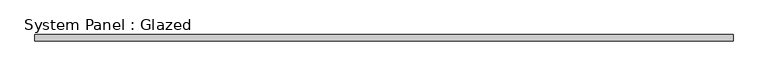
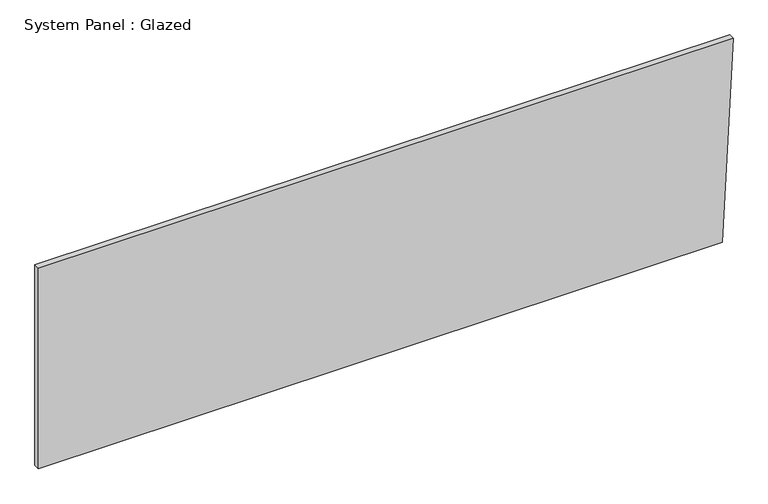
"""IFC4 building model written with IfcOpenShell, lengths in millimetres: plate geometry, System Panel : Glazed."""

import ifcopenshell
import ifcopenshell.guid

model = None  # the IFC model being written
_history = None  # IfcOwnerHistory: only IFC2X3 demands one
_inside = {}  # id of a spatial element -> (the spatial element, [elements in it])
_under = {}  # id of a project, library or spatial element -> (it, [spatial elements below it])
_declared = {}  # id of a project -> (the project, [libraries it declares])
_typed = {}  # id of a type object -> (the type object, [elements of that type])
_made_of = {}  # id of a material, layer set ... -> (it, [elements and type objects made of it])


def new_model(schema):
    """Start an empty IFC model of exactly this schema.

    Asked for "IFC4X3", IfcOpenShell would pick the latest addendum, in which some entities
    have other attributes; the version numbers below select the first issue.
    IFC2X3 requires an IfcOwnerHistory on every rooted entity: one is made here for all.
    """
    global model, _history
    if schema == "IFC4X3":
        model = ifcopenshell.file(schema_version=(4, 3, 0, 0))
    else:
        model = ifcopenshell.file(schema=schema)
    _inside.clear()
    _under.clear()
    _declared.clear()
    _typed.clear()
    _made_of.clear()
    _history = None
    if model.schema == "IFC2X3":
        org = make("IfcOrganization", Name="unknown")
        user = make(
            "IfcPersonAndOrganization",
            ThePerson=make("IfcPerson", FamilyName="unknown"),
            TheOrganization=org,
        )
        app = make(
            "IfcApplication",
            ApplicationDeveloper=org,
            Version="unknown",
            ApplicationFullName="unknown",
            ApplicationIdentifier="unknown",
        )
        _history = make(
            "IfcOwnerHistory",
            OwningUser=user,
            OwningApplication=app,
            ChangeAction="ADDED",
            CreationDate=0,
        )
    return model


def make(cls, **values):
    """One entity of the class cls with the attributes given. An attribute that is None is left unset."""
    return model.create_entity(
        cls, **{name: value for name, value in values.items() if value is not None}
    )


def rooted(cls, **values):
    """An entity with a GlobalId (a new one), such as an element, a storey or a relation."""
    return make(cls, GlobalId=ifcopenshell.guid.new(), OwnerHistory=_history, **values)


def si_unit(unit_type, name, prefix=None):
    """IfcSIUnit, for example si_unit("LENGTHUNIT", "METRE", prefix="MILLI")."""
    return make("IfcSIUnit", UnitType=unit_type, Prefix=prefix, Name=name)


def assignment(units):
    """IfcUnitAssignment: the units of a project."""
    return None if units is None else make("IfcUnitAssignment", Units=units)


def point(xyz):
    """IfcCartesianPoint."""
    return None if xyz is None else make("IfcCartesianPoint", Coordinates=xyz)


def direction(xyz):
    """IfcDirection."""
    return None if xyz is None else make("IfcDirection", DirectionRatios=xyz)


def frame(location, z_axis=None, x_axis=None):
    """IfcAxis2Placement3D, a coordinate frame: its origin and axes. An axis left out is left unset."""
    return make(
        "IfcAxis2Placement3D",
        Location=point(location),
        Axis=direction(z_axis),
        RefDirection=direction(x_axis),
    )


def origin():
    """The frame at (0, 0, 0) with its axes left unset."""
    return frame((0.0, 0.0, 0.0))


def place(relative_to, where):
    """IfcLocalPlacement: puts the frame where relative to a parent placement (None: the world)."""
    return make(
        "IfcLocalPlacement", PlacementRelTo=relative_to, RelativePlacement=where
    )


def context(
    kind, dimensions, precision=None, world=None, true_north=None, identifier=None
):
    """IfcGeometricRepresentationContext, for example the 3D "Model" context."""
    return make(
        "IfcGeometricRepresentationContext",
        ContextIdentifier=identifier,
        ContextType=kind,
        CoordinateSpaceDimension=dimensions,
        Precision=precision,
        WorldCoordinateSystem=world,
        TrueNorth=true_north,
    )


def project(units=None, contexts=None):
    """IfcProject with its units and contexts."""
    return rooted(
        "IfcProject",
        Name="project",
        RepresentationContexts=contexts,
        UnitsInContext=assignment(units),
    )


def spatial(cls, under=None, at=None, **own):
    """A site, building, storey or space (cls), placed at a placement, below another one or the project."""
    s = rooted(cls, ObjectPlacement=at, **own)
    if under is not None:
        _under.setdefault(under.id(), (under, []))[1].append(s)
    return s


def polyline(points):
    """IfcPolyline through the points."""
    return make("IfcPolyline", Points=[point(p) for p in points])


def outline(outer, holes=None, kind="AREA"):
    """IfcArbitraryClosedProfileDef: a profile drawn as a closed curve; with holes, ...WithVoids."""
    if holes is None:
        return make("IfcArbitraryClosedProfileDef", ProfileType=kind, OuterCurve=outer)
    return make(
        "IfcArbitraryProfileDefWithVoids",
        ProfileType=kind,
        OuterCurve=outer,
        InnerCurves=holes,
    )


def extrude(swept, where, along, depth):
    """IfcExtrudedAreaSolid: the profile swept, set in the frame where, extruded along a direction by depth."""
    return make(
        "IfcExtrudedAreaSolid",
        SweptArea=swept,
        Position=where,
        ExtrudedDirection=direction(along),
        Depth=depth,
    )


def shape(context_of_items, identifier, shape_type, items):
    """IfcShapeRepresentation: the items that make up one representation, for example the "Body"."""
    return make(
        "IfcShapeRepresentation",
        ContextOfItems=context_of_items,
        RepresentationIdentifier=identifier,
        RepresentationType=shape_type,
        Items=items,
    )


def source(mapping_origin, context_of_items, identifier, shape_type, items):
    """IfcRepresentationMap: a shape defined once, which mapped items show again and again."""
    return make(
        "IfcRepresentationMap",
        MappingOrigin=mapping_origin,
        MappedRepresentation=shape(context_of_items, identifier, shape_type, items),
    )


def transform(
    local_origin,
    x_axis=None,
    y_axis=None,
    z_axis=None,
    scale=None,
    scale2=None,
    scale3=None,
    uniform=True,
):
    """IfcCartesianTransformationOperator3D, or its non-uniform kind. x_axis, y_axis, z_axis: its Axis1, 2, 3."""
    if uniform:
        return make(
            "IfcCartesianTransformationOperator3D",
            Axis1=direction(x_axis),
            Axis2=direction(y_axis),
            LocalOrigin=point(local_origin),
            Scale=scale,
            Axis3=direction(z_axis),
        )
    return make(
        "IfcCartesianTransformationOperator3DnonUniform",
        Axis1=direction(x_axis),
        Axis2=direction(y_axis),
        LocalOrigin=point(local_origin),
        Scale=scale,
        Axis3=direction(z_axis),
        Scale2=scale2,
        Scale3=scale3,
    )


def mapped(mapping_source, mapping_target):
    """IfcMappedItem: shows the shape of a source again, moved by a transform."""
    return make(
        "IfcMappedItem", MappingSource=mapping_source, MappingTarget=mapping_target
    )


def made_of(thing, what):
    """Note that an element or type object is made of a material, layer set ...; save() writes the relation."""
    if what is not None:
        _made_of.setdefault(what.id(), (what, []))[1].append(thing)
    return thing


def element(
    cls,
    number,
    at=None,
    inside=None,
    cuts=None,
    type_object=None,
    material=None,
    context=None,
    identifier="Body",
    shape_type=None,
    held_by="IfcProductDefinitionShape",
    body=None,
    shapes=None,
    **own,
):
    """One element of the class cls, such as IfcWall. Its Tag is "e" and its number.

    at: its placement. inside: the storey or other place that contains it. cuts: it is an
    opening in that element (IfcRelVoidsElement). A single representation is given by context,
    identifier, shape_type and body (its items); several are given by shapes. held_by: the class
    of the entity that holds the representations. save() writes the other relations.
    """
    e = rooted(cls, Tag="e%d" % number, ObjectPlacement=at, **own)
    if body is not None:
        shapes = [shape(context, identifier, shape_type, body)]
    if shapes is not None:
        e.Representation = make(held_by, Representations=shapes)
    if inside is not None:
        _inside.setdefault(inside.id(), (inside, []))[1].append(e)
    if cuts is not None:
        rooted(
            "IfcRelVoidsElement", RelatingBuildingElement=cuts, RelatedOpeningElement=e
        )
    if type_object is not None:
        _typed.setdefault(type_object.id(), (type_object, []))[1].append(e)
    return made_of(e, material)


def aggregate(whole, parts):
    """IfcRelAggregates: a whole, such as a stair, and the parts it consists of."""
    return rooted("IfcRelAggregates", RelatingObject=whole, RelatedObjects=parts)


def save(model, path):
    """Write the relations noted so far, then the file.

    IfcRelAggregates (storeys below a building ...), IfcRelContainedInSpatialStructure (elements
    in a storey), IfcRelDefinesByType, IfcRelAssociatesMaterial and IfcRelDeclares: one each for
    every whole, place, type object, material and project.
    """
    for whole, parts in _under.values():
        aggregate(whole, parts)
    for where, things in _inside.values():
        rooted(
            "IfcRelContainedInSpatialStructure",
            RelatedElements=things,
            RelatingStructure=where,
        )
    for kind, things in _typed.values():
        rooted("IfcRelDefinesByType", RelatedObjects=things, RelatingType=kind)
    for what, things in _made_of.values():
        rooted("IfcRelAssociatesMaterial", RelatedObjects=things, RelatingMaterial=what)
    for by, libraries in _declared.values():
        rooted("IfcRelDeclares", RelatingContext=by, RelatedDefinitions=libraries)
    model.write(path)


def system_panel_glazed_eafac879(model_context):
    return source(origin(), model_context, "Body", "SweptSolid", [
        extrude(outline(polyline([(0.0, -1421.6824189), (0.0, 1376.3593837), (866.0018549, 1421.6824189), (866.0018549, -1421.6824189), (0.0, -1421.6824189)])), frame((0.0, -44.45, 0.0), z_axis=(0.0, 1.0, 0.0), x_axis=(0.0, 0.0, 1.0)), (0.0, 0.0, 1.0), 25.4),
    ])


if __name__ == "__main__":
    model = new_model("IFC4")
    model_context = context("Model", 3, world=origin())
    ifc_project = project(units=[si_unit("LENGTHUNIT", "METRE", prefix="MILLI")], contexts=[model_context])
    site = spatial("IfcSite", under=ifc_project)
    building = spatial("IfcBuilding", under=site)
    placement = place(None, origin())
    system_panel_glazed_shape = system_panel_glazed_eafac879(model_context)
    element("IfcPlate", 1, ObjectType="System Panel : Glazed", at=placement, inside=building, context=model_context, shape_type="MappedRepresentation", body=[
        mapped(system_panel_glazed_shape, transform((0.0, 0.0, 0.0), x_axis=(1.0, 0.0, 0.0), y_axis=(0.0, 1.0, 0.0), z_axis=(0.0, 0.0, 1.0))),
    ])
    save(model, "model.ifc")

# Revit data of these elements
# Type "System Panel : Glazed"
#   Construction Type Id = "GSP4R"
#   Analytic Construction = "1/8 in Pilkington single glazing"
#   Visual Light Transmittance = 0.9
#   Solar Heat Gain Coefficient = 0.86
#   Heat Transfer Coefficient (U) = 1.18115 BTU/(h·ft²·°F)
#   Define Thermal Properties by = 1
# Element 1 (IfcPlate, "System Panel : Glazed")
#   Materials on its faces: "Glass"
# Materials
#   "Glass": class "Glass", colour RGB 0 128 192, transparency 0.75, Description = "Soda Lime Glass", Cost = 0
